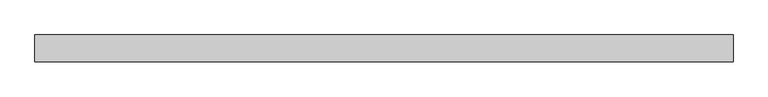
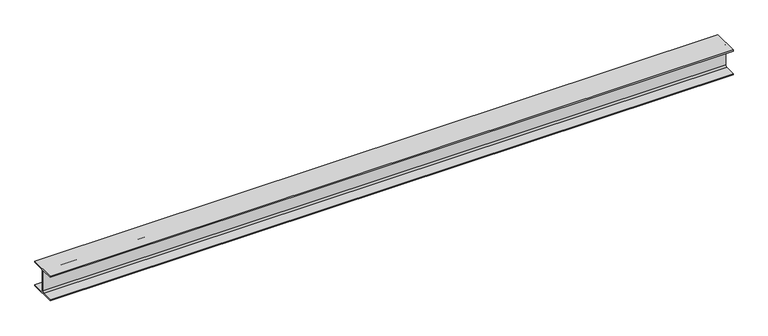
"""IFC4 building model written with IfcOpenShell, lengths in millimetres: beam geometry, 0912_Steel Framing_H-KSD3502 : H_SB_ASB_H-300x300x10x15."""

import ifcopenshell
import ifcopenshell.guid

model = None  # the IFC model being written
_history = None  # IfcOwnerHistory: only IFC2X3 demands one
_inside = {}  # id of a spatial element -> (the spatial element, [elements in it])
_under = {}  # id of a project, library or spatial element -> (it, [spatial elements below it])
_declared = {}  # id of a project -> (the project, [libraries it declares])
_typed = {}  # id of a type object -> (the type object, [elements of that type])
_made_of = {}  # id of a material, layer set ... -> (it, [elements and type objects made of it])


def new_model(schema):
    """Start an empty IFC model of exactly this schema.

    Asked for "IFC4X3", IfcOpenShell would pick the latest addendum, in which some entities
    have other attributes; the version numbers below select the first issue.
    IFC2X3 requires an IfcOwnerHistory on every rooted entity: one is made here for all.
    """
    global model, _history
    if schema == "IFC4X3":
        model = ifcopenshell.file(schema_version=(4, 3, 0, 0))
    else:
        model = ifcopenshell.file(schema=schema)
    _inside.clear()
    _under.clear()
    _declared.clear()
    _typed.clear()
    _made_of.clear()
    _history = None
    if model.schema == "IFC2X3":
        org = make("IfcOrganization", Name="unknown")
        user = make(
            "IfcPersonAndOrganization",
            ThePerson=make("IfcPerson", FamilyName="unknown"),
            TheOrganization=org,
        )
        app = make(
            "IfcApplication",
            ApplicationDeveloper=org,
            Version="unknown",
            ApplicationFullName="unknown",
            ApplicationIdentifier="unknown",
        )
        _history = make(
            "IfcOwnerHistory",
            OwningUser=user,
            OwningApplication=app,
            ChangeAction="ADDED",
            CreationDate=0,
        )
    return model


def make(cls, **values):
    """One entity of the class cls with the attributes given. An attribute that is None is left unset."""
    return model.create_entity(
        cls, **{name: value for name, value in values.items() if value is not None}
    )


def rooted(cls, **values):
    """An entity with a GlobalId (a new one), such as an element, a storey or a relation."""
    return make(cls, GlobalId=ifcopenshell.guid.new(), OwnerHistory=_history, **values)


def si_unit(unit_type, name, prefix=None):
    """IfcSIUnit, for example si_unit("LENGTHUNIT", "METRE", prefix="MILLI")."""
    return make("IfcSIUnit", UnitType=unit_type, Prefix=prefix, Name=name)


def assignment(units):
    """IfcUnitAssignment: the units of a project."""
    return None if units is None else make("IfcUnitAssignment", Units=units)


def point(xyz):
    """IfcCartesianPoint."""
    return None if xyz is None else make("IfcCartesianPoint", Coordinates=xyz)


def direction(xyz):
    """IfcDirection."""
    return None if xyz is None else make("IfcDirection", DirectionRatios=xyz)


def frame(location, z_axis=None, x_axis=None):
    """IfcAxis2Placement3D, a coordinate frame: its origin and axes. An axis left out is left unset."""
    return make(
        "IfcAxis2Placement3D",
        Location=point(location),
        Axis=direction(z_axis),
        RefDirection=direction(x_axis),
    )


def frame_2d(location, x_axis=None):
    """IfcAxis2Placement2D, a coordinate frame in the plane: its origin and x axis."""
    return make(
        "IfcAxis2Placement2D", Location=point(location), RefDirection=direction(x_axis)
    )


def origin():
    """The frame at (0, 0, 0) with its axes left unset."""
    return frame((0.0, 0.0, 0.0))


def place(relative_to, where):
    """IfcLocalPlacement: puts the frame where relative to a parent placement (None: the world)."""
    return make(
        "IfcLocalPlacement", PlacementRelTo=relative_to, RelativePlacement=where
    )


def context(
    kind, dimensions, precision=None, world=None, true_north=None, identifier=None
):
    """IfcGeometricRepresentationContext, for example the 3D "Model" context."""
    return make(
        "IfcGeometricRepresentationContext",
        ContextIdentifier=identifier,
        ContextType=kind,
        CoordinateSpaceDimension=dimensions,
        Precision=precision,
        WorldCoordinateSystem=world,
        TrueNorth=true_north,
    )


def project(units=None, contexts=None):
    """IfcProject with its units and contexts."""
    return rooted(
        "IfcProject",
        Name="project",
        RepresentationContexts=contexts,
        UnitsInContext=assignment(units),
    )


def spatial(cls, under=None, at=None, **own):
    """A site, building, storey or space (cls), placed at a placement, below another one or the project."""
    s = rooted(cls, ObjectPlacement=at, **own)
    if under is not None:
        _under.setdefault(under.id(), (under, []))[1].append(s)
    return s


def polyline(points):
    """IfcPolyline through the points."""
    return make("IfcPolyline", Points=[point(p) for p in points])


def circle_curve(where, radius):
    """IfcCircle in the frame where."""
    return make("IfcCircle", Position=where, Radius=radius)


def trimmed(basis, trim1, trim2, sense, master):
    """IfcTrimmedCurve: the piece of a basis curve between two trims."""
    return make(
        "IfcTrimmedCurve",
        BasisCurve=basis,
        Trim1=trim1,
        Trim2=trim2,
        SenseAgreement=sense,
        MasterRepresentation=master,
    )


def segment(curve, same_sense, transition):
    """IfcCompositeCurveSegment."""
    return make(
        "IfcCompositeCurveSegment",
        Transition=transition,
        SameSense=same_sense,
        ParentCurve=curve,
    )


def composite_curve(segments, self_intersect=None):
    """IfcCompositeCurve: segments joined end to end."""
    return make("IfcCompositeCurve", Segments=segments, SelfIntersect=self_intersect)


def outline(outer, holes=None, kind="AREA"):
    """IfcArbitraryClosedProfileDef: a profile drawn as a closed curve; with holes, ...WithVoids."""
    if holes is None:
        return make("IfcArbitraryClosedProfileDef", ProfileType=kind, OuterCurve=outer)
    return make(
        "IfcArbitraryProfileDefWithVoids",
        ProfileType=kind,
        OuterCurve=outer,
        InnerCurves=holes,
    )


def extrude(swept, where, along, depth):
    """IfcExtrudedAreaSolid: the profile swept, set in the frame where, extruded along a direction by depth."""
    return make(
        "IfcExtrudedAreaSolid",
        SweptArea=swept,
        Position=where,
        ExtrudedDirection=direction(along),
        Depth=depth,
    )


def shape(context_of_items, identifier, shape_type, items):
    """IfcShapeRepresentation: the items that make up one representation, for example the "Body"."""
    return make(
        "IfcShapeRepresentation",
        ContextOfItems=context_of_items,
        RepresentationIdentifier=identifier,
        RepresentationType=shape_type,
        Items=items,
    )


def source(mapping_origin, context_of_items, identifier, shape_type, items):
    """IfcRepresentationMap: a shape defined once, which mapped items show again and again."""
    return make(
        "IfcRepresentationMap",
        MappingOrigin=mapping_origin,
        MappedRepresentation=shape(context_of_items, identifier, shape_type, items),
    )


def transform(
    local_origin,
    x_axis=None,
    y_axis=None,
    z_axis=None,
    scale=None,
    scale2=None,
    scale3=None,
    uniform=True,
):
    """IfcCartesianTransformationOperator3D, or its non-uniform kind. x_axis, y_axis, z_axis: its Axis1, 2, 3."""
    if uniform:
        return make(
            "IfcCartesianTransformationOperator3D",
            Axis1=direction(x_axis),
            Axis2=direction(y_axis),
            LocalOrigin=point(local_origin),
            Scale=scale,
            Axis3=direction(z_axis),
        )
    return make(
        "IfcCartesianTransformationOperator3DnonUniform",
        Axis1=direction(x_axis),
        Axis2=direction(y_axis),
        LocalOrigin=point(local_origin),
        Scale=scale,
        Axis3=direction(z_axis),
        Scale2=scale2,
        Scale3=scale3,
    )


def mapped(mapping_source, mapping_target):
    """IfcMappedItem: shows the shape of a source again, moved by a transform."""
    return make(
        "IfcMappedItem", MappingSource=mapping_source, MappingTarget=mapping_target
    )


def made_of(thing, what):
    """Note that an element or type object is made of a material, layer set ...; save() writes the relation."""
    if what is not None:
        _made_of.setdefault(what.id(), (what, []))[1].append(thing)
    return thing


def element(
    cls,
    number,
    at=None,
    inside=None,
    cuts=None,
    type_object=None,
    material=None,
    context=None,
    identifier="Body",
    shape_type=None,
    held_by="IfcProductDefinitionShape",
    body=None,
    shapes=None,
    **own,
):
    """One element of the class cls, such as IfcWall. Its Tag is "e" and its number.

    at: its placement. inside: the storey or other place that contains it. cuts: it is an
    opening in that element (IfcRelVoidsElement). A single representation is given by context,
    identifier, shape_type and body (its items); several are given by shapes. held_by: the class
    of the entity that holds the representations. save() writes the other relations.
    """
    e = rooted(cls, Tag="e%d" % number, ObjectPlacement=at, **own)
    if body is not None:
        shapes = [shape(context, identifier, shape_type, body)]
    if shapes is not None:
        e.Representation = make(held_by, Representations=shapes)
    if inside is not None:
        _inside.setdefault(inside.id(), (inside, []))[1].append(e)
    if cuts is not None:
        rooted(
            "IfcRelVoidsElement", RelatingBuildingElement=cuts, RelatedOpeningElement=e
        )
    if type_object is not None:
        _typed.setdefault(type_object.id(), (type_object, []))[1].append(e)
    return made_of(e, material)


def aggregate(whole, parts):
    """IfcRelAggregates: a whole, such as a stair, and the parts it consists of."""
    return rooted("IfcRelAggregates", RelatingObject=whole, RelatedObjects=parts)


def save(model, path):
    """Write the relations noted so far, then the file.

    IfcRelAggregates (storeys below a building ...), IfcRelContainedInSpatialStructure (elements
    in a storey), IfcRelDefinesByType, IfcRelAssociatesMaterial and IfcRelDeclares: one each for
    every whole, place, type object, material and project.
    """
    for whole, parts in _under.values():
        aggregate(whole, parts)
    for where, things in _inside.values():
        rooted(
            "IfcRelContainedInSpatialStructure",
            RelatedElements=things,
            RelatingStructure=where,
        )
    for kind, things in _typed.values():
        rooted("IfcRelDefinesByType", RelatedObjects=things, RelatingType=kind)
    for what, things in _made_of.values():
        rooted("IfcRelAssociatesMaterial", RelatedObjects=things, RelatingMaterial=what)
    for by, libraries in _declared.values():
        rooted("IfcRelDeclares", RelatingContext=by, RelatedDefinitions=libraries)
    model.write(path)


def beam_8c8e336d(model_context):
    return source(origin(), model_context, "Body", "SweptSolid", [
        extrude(outline(composite_curve([segment(polyline([(150.0, -135.0), (150.0, -150.0), (-150.0, -150.0), (-150.0, -135.0), (-23.0, -135.0)]), True, "CONTINUOUS"), segment(trimmed(circle_curve(frame_2d((-23.0, -117.0)), 18.0), [point((-23.0, -135.0))], [point((-5.0, -117.0))], True, "CARTESIAN"), True, "CONTINUOUS"), segment(polyline([(-5.0, -117.0), (-5.0, 117.0)]), True, "CONTINUOUS"), segment(trimmed(circle_curve(frame_2d((-23.0, 117.0)), 18.0), [point((-5.0, 117.0))], [point((-23.0, 135.0))], True, "CARTESIAN"), True, "CONTINUOUS"), segment(polyline([(-23.0, 135.0), (-150.0, 135.0), (-150.0, 150.0), (150.0, 150.0), (150.0, 135.0), (23.0, 135.0)]), True, "CONTINUOUS"), segment(trimmed(circle_curve(frame_2d((23.0, 117.0)), 18.0), [point((23.0, 135.0))], [point((5.0, 117.0))], True, "CARTESIAN"), True, "CONTINUOUS"), segment(polyline([(5.0, 117.0), (5.0, -117.0)]), True, "CONTINUOUS"), segment(trimmed(circle_curve(frame_2d((23.0, -117.0)), 18.0), [point((5.0, -117.0))], [point((23.0, -135.0))], True, "CARTESIAN"), True, "CONTINUOUS"), segment(polyline([(23.0, -135.0), (150.0, -135.0)]), True, "CONTINUOUS")], self_intersect=False)), frame((-4027.4502484, 0.0, 0.0), z_axis=(1.0, 0.0, 0.0), x_axis=(0.0, 1.0, 0.0)), (0.0, 0.0, 1.0), 7805.3816456),
    ])


if __name__ == "__main__":
    model = new_model("IFC4")
    model_context = context("Model", 3, world=origin())
    ifc_project = project(units=[si_unit("LENGTHUNIT", "METRE", prefix="MILLI")], contexts=[model_context])
    site = spatial("IfcSite", under=ifc_project)
    building = spatial("IfcBuilding", under=site)
    placement = place(None, origin())
    beam_shape = beam_8c8e336d(model_context)
    element("IfcBeam", 1, ObjectType="0912_Steel Framing_H-KSD3502 : H_SB_ASB_H-300x300x10x15", at=placement, inside=building, context=model_context, shape_type="MappedRepresentation", body=[
        mapped(beam_shape, transform((0.0, 0.0, 0.0), x_axis=(1.0, 0.0, 0.0), y_axis=(0.0, 1.0, 0.0), z_axis=(0.0, 0.0, 1.0))),
    ])
    save(model, "model.ifc")

# Revit data of these elements
# Type "0912_Steel Framing_H-KSD3502 : H_SB_ASB_H-300x300x10x15"
#   H_WM Code_1 = "S01AA001-00001 | Main Steel Structure Fabrication Work | Shelter/Building | Heavy Steel - Standard (Weight≥90KG/M) | Material: (   )"
#   H_WM Code_2 = "S03AA027-00001 | Main Steel Structure Erection Work | Shelter/Building | Heavy Steel (Weight≥90KG/M) | Material: (   )"
#   H_WM Code_3 = "S01AA010-00001 | Main Steel Structure Fabrication Work | Shelter/Building | Steel Painting/Coating | for Non-Fireproofed Steel Surface, Surface Preparation, Primer, Second & Final Coat | Material: (   )"
#   H_Q'ty Cal Type Tag = "SB-Q2"
#   Width = 30.0 cm
#   Web Thickness = 1.0 cm
#   Web Fillet = 1.8 cm
#   Warping Constant = 1370000.0 cm⁶
#   W = 0
#   Torsional Moment of Inertia = 77.00 cm⁴
#   Section Area = 119.8 cm²
#   Plastic Modulus weak axis = 684.0 cm³
#   Plastic Modulus strong axis = 1500.0 cm³
#   Perimeter = 1.75 m²/m
#   Nominal Weight = 94.00 kgf/m
#   Moment of Inertia weak axis = 6750.00 cm⁴
#   Moment of Inertia strong axis = 20400.00 cm⁴
#   Height = 30.0 cm
#   Flange Thickness = 1.5 cm
#   Elastic Modulus weak axis = 450.0 cm³
#   Elastic Modulus strong axis = 1360.0 cm³
#   Centroid Vertical = 15.0 cm
#   Centroid Horizontal = 15.0 cm
#   Ix = 204000000
#   Length [instance default] = 1.5240 m
#   Zx = 1500000
#   b = 0.3000 m
#   h = 0.3000 m
#   r = 0.0180 m
#   s = 0.0100 m
#   t = 0.0150 m
#   A = 0.01198 m²
#   Structural Material [instance default] = Steel, 45-345
#   Assembly Code = ""
# Element 1 (IfcBeam, "0912_Steel Framing_H-KSD3502 : H_SB_ASB_H-300x300x10x15")
#   Structural Material = none
# Materials
#   "Steel, 45-345": class "Metal", colour RGB 189 187 185, transparency 0, Description = "Steel 345 MPa", Cost = 0
